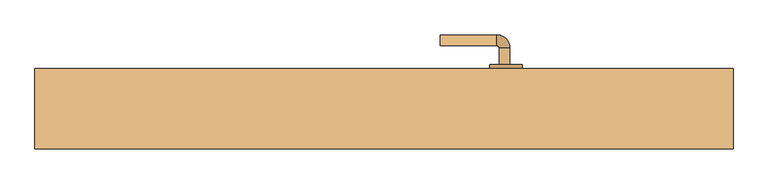
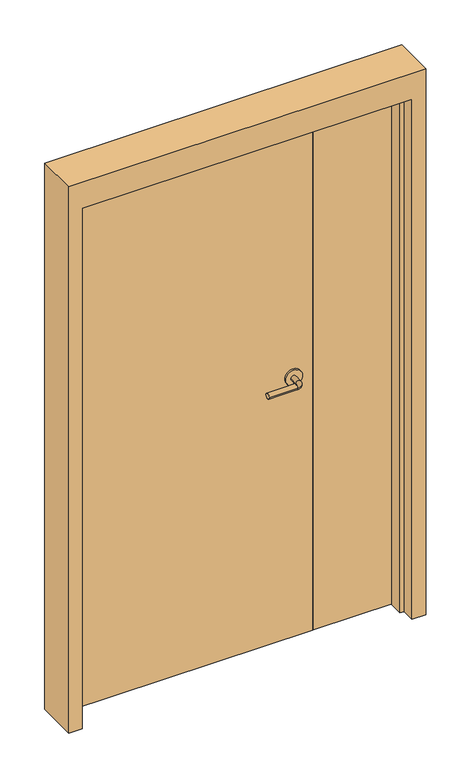
"""IFC4 building model written with IfcOpenShell, lengths in millimetres: door geometry, Дверь-Маятниковая-С полотнами разной ширины-Щитовая : 1300 x 2100 мм."""

from ifc_helpers import new_model, si_unit, point, frame, frame_2d, origin, origin_with_axes, place, context, project, spatial, polyline, circle_curve, ellipse_curve, trimmed, segment, composite_curve, outline, extrude, faceted_brep, source, transform, mapped, element, save
from ifc_brep_helpers import plane_surface, cylinder_surface, revolved_surface, advanced_brep


def door_c0d84948(model_context):
    return source(origin(), model_context, "Body", "SolidModel", [
        advanced_brep(
        [(234.59375, 15.85, 1000.0), (214.59375, 15.85, 1000.0), (234.59375, -14.15, 1000.0), (214.59375, -14.15, 1000.0), (209.59375, -19.15, 1000.0), (209.59375, -39.15, 1000.0), (104.59375, -39.15, 1000.0), (104.59375, -19.15, 1000.0)],
        [
            (0, 1, circle_curve(frame((224.59375, 15.85, 1000.0), z_axis=(0.0, 1.0, 0.0), x_axis=(-1.0, 0.0, 0.0)), 10.0)),
            (1, 0, circle_curve(frame((224.59375, 15.85, 1000.0), z_axis=(0.0, 1.0, 0.0), x_axis=(-1.0, 0.0, 0.0)), 10.0)),
            (0, 2),
            (2, 3, circle_curve(frame((224.59375, -14.15, 1000.0), z_axis=(0.0, 1.0, 0.0), x_axis=(-1.0, 0.0, 0.0)), 10.0)),
            (3, 1),
            (3, 2, circle_curve(frame((224.59375, -14.15, 1000.0), z_axis=(0.0, 1.0, 0.0), x_axis=(-1.0, 0.0, 0.0)), 10.0)),
            (4, 3, circle_curve(frame((209.59375, -14.15, 1000.0), z_axis=(0.0, 0.0, 1.0), x_axis=(1.0, 0.0, 0.0)), 5.0)),
            (2, 5, circle_curve(frame((209.59375, -14.15, 1000.0), z_axis=(0.0, 0.0, -1.0), x_axis=(1.0, 0.0, 0.0)), 25.0)),
            (5, 4, circle_curve(frame((209.59375, -29.15, 1000.0), z_axis=(1.0, 0.0, 0.0), x_axis=(0.0, 1.0, 0.0)), 10.0)),
            (4, 5, circle_curve(frame((209.59375, -29.15, 1000.0), z_axis=(1.0, 0.0, 0.0), x_axis=(0.0, 1.0, 0.0)), 10.0)),
            (6, 7, circle_curve(frame((104.59375, -29.15, 1000.0), z_axis=(-1.0, 0.0, 0.0), x_axis=(0.0, 1.0, 0.0)), 10.0)),
            (7, 6, circle_curve(frame((104.59375, -29.15, 1000.0), z_axis=(-1.0, 0.0, 0.0), x_axis=(0.0, 1.0, 0.0)), 10.0)),
            (5, 6),
            (7, 4),
        ],
        [
            plane_surface(frame((224.59375, 15.85, 1000.0), z_axis=(0.0, 1.0, 0.0), x_axis=(0.0, 0.0, 1.0))),
            cylinder_surface(frame((224.59375, 15.85, 1000.0), z_axis=(0.0, 1.0, 0.0), x_axis=(-1.0, 0.0, 0.0)), 10.0),
            revolved_surface(trimmed(ellipse_curve(frame((224.59375, -14.15, 1000.0), z_axis=(0.0, 1.0, 0.0), x_axis=(-1.0, 0.0, 0.0)), 10.0, 10.0), [point((234.59375, -14.15, 1000.0))], [point((214.59375, -14.15, 1000.0))], True, "CARTESIAN"), (209.59375, -14.15, 1000.0), (0.0, 0.0, -1.0)),
            revolved_surface(trimmed(ellipse_curve(frame((224.59375, -14.15, 1000.0), z_axis=(0.0, 1.0, 0.0), x_axis=(-1.0, 0.0, 0.0)), 10.0, 10.0), [point((214.59375, -14.15, 1000.0))], [point((234.59375, -14.15, 1000.0))], True, "CARTESIAN"), (209.59375, -14.15, 1000.0), (0.0, 0.0, -1.0)),
            plane_surface(frame((104.59375, -29.15, 1000.0), z_axis=(-1.0, 0.0, 0.0), x_axis=(0.0, 0.0, 1.0))),
            cylinder_surface(frame((209.59375, -29.15, 1000.0), z_axis=(1.0, 0.0, 0.0), x_axis=(0.0, 1.0, 0.0)), 10.0),
        ],
        [
            (0, [[1, 2]]),
            (1, [[-1, 3, 4, 5]]),
            (1, [[-2, -5, 6, -3]]),
            (2, [[7, -4, 8, 9]]),
            (3, [[-8, -6, -7, 10]]),
            (4, [[11, 12]]),
            (5, [[-9, 13, -12, 14]]),
            (5, [[-10, -14, -11, -13]]),
        ],
    ),
        extrude(outline(composite_curve([segment(trimmed(circle_curve(frame_2d((1000.0, 227.09375)), 30.0), [point((1000.0, 257.09375))], [point((1000.0, 197.09375))], False, "CARTESIAN"), True, "CONTINUOUS"), segment(trimmed(circle_curve(frame_2d((1000.0, 227.09375)), 30.0), [point((1000.0, 197.09375))], [point((1000.0, 257.09375))], False, "CARTESIAN"), True, "CONTINUOUS")], self_intersect=False)), frame((0.0, 15.85, 0.0), z_axis=(0.0, 1.0, 0.0), x_axis=(0.0, 0.0, 1.0)), (0.0, 0.0, 1.0), 8.0),
        advanced_brep(
        [(234.59375, 76.85, 1000.0), (214.59375, 76.85, 1000.0), (214.59375, 106.85, 1000.0), (234.59375, 106.85, 1000.0), (209.59375, 111.85, 1000.0), (209.59375, 131.85, 1000.0), (104.59375, 131.85, 1000.0), (104.59375, 111.85, 1000.0)],
        [
            (0, 1, circle_curve(frame((224.59375, 76.85, 1000.0), z_axis=(0.0, -1.0, 0.0), x_axis=(-1.0, 0.0, 0.0)), 10.0)),
            (1, 0, circle_curve(frame((224.59375, 76.85, 1000.0), z_axis=(0.0, -1.0, 0.0), x_axis=(-1.0, 0.0, 0.0)), 10.0)),
            (1, 2),
            (2, 3, circle_curve(frame((224.59375, 106.85, 1000.0), z_axis=(0.0, -1.0, 0.0), x_axis=(-1.0, 0.0, 0.0)), 10.0)),
            (3, 0),
            (3, 2, circle_curve(frame((224.59375, 106.85, 1000.0), z_axis=(0.0, -1.0, 0.0), x_axis=(-1.0, 0.0, 0.0)), 10.0)),
            (4, 5, circle_curve(frame((209.59375, 121.85, 1000.0), z_axis=(1.0, 0.0, 0.0), x_axis=(0.0, -1.0, 0.0)), 10.0)),
            (5, 3, circle_curve(frame((209.59375, 106.85, 1000.0), z_axis=(0.0, 0.0, -1.0), x_axis=(1.0, 0.0, 0.0)), 25.0)),
            (2, 4, circle_curve(frame((209.59375, 106.85, 1000.0), z_axis=(0.0, 0.0, 1.0), x_axis=(1.0, 0.0, 0.0)), 5.0)),
            (5, 4, circle_curve(frame((209.59375, 121.85, 1000.0), z_axis=(1.0, 0.0, 0.0), x_axis=(0.0, -1.0, 0.0)), 10.0)),
            (6, 7, circle_curve(frame((104.59375, 121.85, 1000.0), z_axis=(-1.0, 0.0, 0.0), x_axis=(0.0, -1.0, 0.0)), 10.0)),
            (7, 6, circle_curve(frame((104.59375, 121.85, 1000.0), z_axis=(-1.0, 0.0, 0.0), x_axis=(0.0, -1.0, 0.0)), 10.0)),
            (4, 7),
            (6, 5),
        ],
        [
            plane_surface(frame((224.59375, 76.85, 1000.0), z_axis=(0.0, -1.0, 0.0), x_axis=(0.0, 0.0, 1.0))),
            cylinder_surface(frame((224.59375, 76.85, 1000.0), z_axis=(0.0, -1.0, 0.0), x_axis=(-1.0, 0.0, 0.0)), 10.0),
            revolved_surface(trimmed(ellipse_curve(frame((224.59375, 106.85, 1000.0), z_axis=(0.0, 1.0, 0.0), x_axis=(-1.0, 0.0, 0.0)), 10.0, 10.0), [point((234.59375, 106.85, 1000.0))], [point((214.59375, 106.85, 1000.0))], True, "CARTESIAN"), (209.59375, 106.85, 1000.0), (0.0, 0.0, -1.0)),
            revolved_surface(trimmed(ellipse_curve(frame((224.59375, 106.85, 1000.0), z_axis=(0.0, 1.0, 0.0), x_axis=(-1.0, 0.0, 0.0)), 10.0, 10.0), [point((214.59375, 106.85, 1000.0))], [point((234.59375, 106.85, 1000.0))], True, "CARTESIAN"), (209.59375, 106.85, 1000.0), (0.0, 0.0, -1.0)),
            plane_surface(frame((104.59375, 121.85, 1000.0), z_axis=(-1.0, 0.0, 0.0), x_axis=(0.0, 0.0, 1.0))),
            cylinder_surface(frame((209.59375, 121.85, 1000.0), z_axis=(1.0, 0.0, 0.0), x_axis=(0.0, -1.0, 0.0)), 10.0),
        ],
        [
            (0, [[1, 2]]),
            (1, [[3, 4, 5, -2]]),
            (1, [[-5, 6, -3, -1]]),
            (2, [[7, 8, -4, 9]]),
            (3, [[10, -9, -6, -8]]),
            (4, [[11, 12]]),
            (5, [[13, -11, 14, -7]]),
            (5, [[-14, -12, -13, -10]]),
        ],
    ),
        extrude(outline(composite_curve([segment(trimmed(circle_curve(frame_2d((1000.0, 227.09375)), 30.0), [point((1000.0, 257.09375))], [point((1000.0, 197.09375))], False, "CARTESIAN"), True, "CONTINUOUS"), segment(trimmed(circle_curve(frame_2d((1000.0, 227.09375)), 30.0), [point((1000.0, 197.09375))], [point((1000.0, 257.09375))], False, "CARTESIAN"), True, "CONTINUOUS")], self_intersect=False)), frame((0.0, 68.85, 0.0), z_axis=(0.0, 1.0, 0.0), x_axis=(0.0, 0.0, 1.0)), (0.0, 0.0, 1.0), 8.0),
        extrude(outline(polyline([(600.0, 23.85), (301.6, 23.85), (301.6, 68.85), (600.0, 68.85), (600.0, 23.85)])), origin_with_axes(), (0.0, 0.0, 1.0), 2000.0),
        faceted_brep([(600.0, 19.0875, 0.0), (600.0, 68.85, 0.0), (650.0, 68.85, 0.0), (650.0, -81.15, 0.0), (600.0, -81.15, 0.0), (600.0, -31.9375, 0.0), (584.125, -31.9375, 0.0), (584.125, 19.0875, 0.0), (600.0, 19.0875, 2000.0), (600.0, 68.85, 2000.0), (-600.0, 68.85, 2000.0), (-600.0, 68.85, 0.0), (-650.0, 68.85, 0.0), (-650.0, 68.85, 2100.0), (650.0, 68.85, 2100.0), (650.0, -81.15, 2100.0), (-650.0, -81.15, 2100.0), (-650.0, -81.15, 0.0), (-600.0, -81.15, 0.0), (-600.0, -81.15, 2000.0), (600.0, -81.15, 2000.0), (600.0, -31.9375, 2000.0), (-600.0, -31.9375, 2000.0), (-600.0, -31.9375, 0.0), (-584.125, -31.9375, 0.0), (-584.125, -31.9375, 1984.125), (584.125, -31.9375, 1984.125), (584.125, 19.0875, 1984.125), (-584.125, 19.0875, 1984.125), (-584.125, 19.0875, 0.0), (-600.0, 19.0875, 0.0), (-600.0, 19.0875, 2000.0)], [[[0, 1, 2, 3, 4, 5, 6, 7]], [[1, 0, 8, 9]], [[2, 1, 9, 10, 11, 12, 13, 14]], [[3, 2, 14, 15]], [[4, 3, 15, 16, 17, 18, 19, 20]], [[5, 4, 20, 21]], [[6, 5, 21, 22, 23, 24, 25, 26]], [[7, 6, 26, 27]], [[0, 7, 27, 28, 29, 30, 31, 8]], [[9, 8, 31, 10]], [[20, 19, 22, 21]], [[26, 25, 28, 27]], [[12, 11, 30, 29, 24, 23, 18, 17]], [[11, 10, 31, 30]], [[13, 12, 17, 16]], [[19, 18, 23, 22]], [[25, 24, 29, 28]], [[15, 14, 13, 16]]]),
        extrude(outline(polyline([(298.4, 23.85), (-600.0, 23.85), (-600.0, 68.85), (298.4, 68.85), (298.4, 23.85)])), origin_with_axes(), (0.0, 0.0, 1.0), 2000.0),
    ])


if __name__ == "__main__":
    model = new_model("IFC4")
    model_context = context("Model", 3, world=origin())
    ifc_project = project(units=[si_unit("LENGTHUNIT", "METRE", prefix="MILLI")], contexts=[model_context])
    site = spatial("IfcSite", under=ifc_project)
    building = spatial("IfcBuilding", under=site)
    placement = place(None, origin())
    door_shape = door_c0d84948(model_context)
    element("IfcDoor", 1, ObjectType="Дверь-Маятниковая-С полотнами разной ширины-Щитовая : 1300 x 2100 мм", at=placement, inside=building, context=model_context, shape_type="MappedRepresentation", body=[
        mapped(door_shape, transform((0.0, 0.0, 0.0), x_axis=(1.0, 0.0, 0.0), y_axis=(0.0, 1.0, 0.0), z_axis=(0.0, 0.0, 1.0))),
    ])
    save(model, "model.ifc")

# Revit data of these elements
# Type "Дверь-Маятниковая-С полотнами разной ширины-Щитовая : 1300 x 2100 мм"
#   Type Mark = "144"
#   Assembly Code = "C1020300"
#   Analytic Construction = "Деревянный"
#   Ширина большой панели = 900 mm
#   W = 300 mm
#   Thickness = 45 mm
#   Thermal Resistance (R) = 0.455703 (m²·K)/W
#   Угол поворота [instance default] = 90°
#   Высота планки = 1000 mm
#   Rough Width [instance default] = 1300 mm
#   Rough Height [instance default] = 2100 mm
#   Высота проема в кирпичном каркасе [instance default] = 100 mm
#   Ширина проема в кирпичном каркасе [instance default] = 100 mm
#   Расчет вставки [instance default] = 105 mm
#   Кирпичная вставка [instance default] = 25 mm
#   Height = 2000 mm
#   Width = 1200 mm
#   Heat Transfer Coefficient (U) = 2.19465 W/(m²·K)
#   Глубина кирпичного каркаса = 150 mm
#   Кирпичный каркас [instance default] = yes
#   Каркас стены сухой кладки [instance default] = no
#   Материал панели = Древесина - Береза
#   Материал каркаса = Металл - Окрашенный - Серый 2
#   Материал дверной ручки = Алюминий
#   Visual Light Transmittance = 0
#   Solar Heat Gain Coefficient = 0
#   Wall Closure = (empty or 0)
#   Function = (empty or 0)
# Element 1 (IfcDoor, "Дверь-Маятниковая-С полотнами разной ширины-Щитовая : 1300 x 2100 мм")
#   Расчет вставки = 80 mm
#   Кирпичная вставка = 0 mm
#   Materials on its faces: "Алюминий", "Металл - Окрашенный - Серый 2", "Древесина - Береза"
# Materials
#   "Древесина - Береза": class "Древесина", colour RGB 166 116 52, transparency 0, Cost = 0
#   "Металл - Окрашенный - Серый 2": class "Краска", colour RGB 104 104 104, transparency 0, Cost = 0
#   "Алюминий": class "Металл", colour RGB 247 247 247, transparency 0
